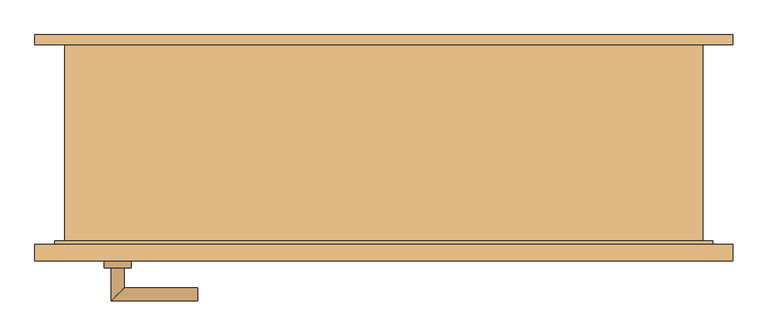
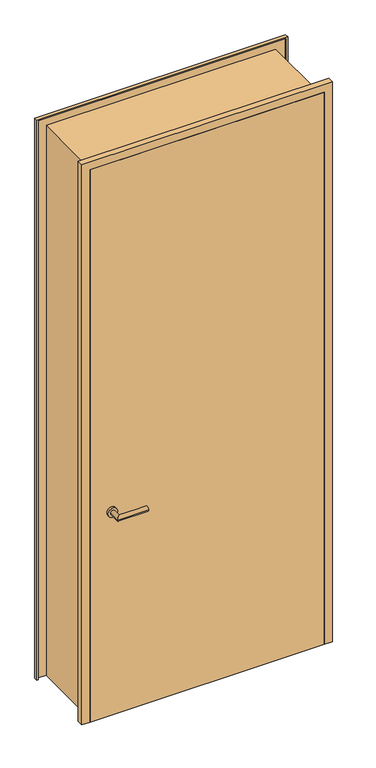
"""IFC4 building model written with IfcOpenShell, lengths in millimetres: door geometry, Drehflügel 1-flg - Stahlzarge : Holztüre 1,0 x 2,45."""

import ifcopenshell
import ifcopenshell.guid

model = None  # the IFC model being written
_history = None  # IfcOwnerHistory: only IFC2X3 demands one
_inside = {}  # id of a spatial element -> (the spatial element, [elements in it])
_under = {}  # id of a project, library or spatial element -> (it, [spatial elements below it])
_declared = {}  # id of a project -> (the project, [libraries it declares])
_typed = {}  # id of a type object -> (the type object, [elements of that type])
_made_of = {}  # id of a material, layer set ... -> (it, [elements and type objects made of it])


def new_model(schema):
    """Start an empty IFC model of exactly this schema.

    Asked for "IFC4X3", IfcOpenShell would pick the latest addendum, in which some entities
    have other attributes; the version numbers below select the first issue.
    IFC2X3 requires an IfcOwnerHistory on every rooted entity: one is made here for all.
    """
    global model, _history
    if schema == "IFC4X3":
        model = ifcopenshell.file(schema_version=(4, 3, 0, 0))
    else:
        model = ifcopenshell.file(schema=schema)
    _inside.clear()
    _under.clear()
    _declared.clear()
    _typed.clear()
    _made_of.clear()
    _history = None
    if model.schema == "IFC2X3":
        org = make("IfcOrganization", Name="unknown")
        user = make(
            "IfcPersonAndOrganization",
            ThePerson=make("IfcPerson", FamilyName="unknown"),
            TheOrganization=org,
        )
        app = make(
            "IfcApplication",
            ApplicationDeveloper=org,
            Version="unknown",
            ApplicationFullName="unknown",
            ApplicationIdentifier="unknown",
        )
        _history = make(
            "IfcOwnerHistory",
            OwningUser=user,
            OwningApplication=app,
            ChangeAction="ADDED",
            CreationDate=0,
        )
    return model


def make(cls, **values):
    """One entity of the class cls with the attributes given. An attribute that is None is left unset."""
    return model.create_entity(
        cls, **{name: value for name, value in values.items() if value is not None}
    )


def rooted(cls, **values):
    """An entity with a GlobalId (a new one), such as an element, a storey or a relation."""
    return make(cls, GlobalId=ifcopenshell.guid.new(), OwnerHistory=_history, **values)


def si_unit(unit_type, name, prefix=None):
    """IfcSIUnit, for example si_unit("LENGTHUNIT", "METRE", prefix="MILLI")."""
    return make("IfcSIUnit", UnitType=unit_type, Prefix=prefix, Name=name)


def assignment(units):
    """IfcUnitAssignment: the units of a project."""
    return None if units is None else make("IfcUnitAssignment", Units=units)


def point(xyz):
    """IfcCartesianPoint."""
    return None if xyz is None else make("IfcCartesianPoint", Coordinates=xyz)


def direction(xyz):
    """IfcDirection."""
    return None if xyz is None else make("IfcDirection", DirectionRatios=xyz)


def frame(location, z_axis=None, x_axis=None):
    """IfcAxis2Placement3D, a coordinate frame: its origin and axes. An axis left out is left unset."""
    return make(
        "IfcAxis2Placement3D",
        Location=point(location),
        Axis=direction(z_axis),
        RefDirection=direction(x_axis),
    )


def frame_2d(location, x_axis=None):
    """IfcAxis2Placement2D, a coordinate frame in the plane: its origin and x axis."""
    return make(
        "IfcAxis2Placement2D", Location=point(location), RefDirection=direction(x_axis)
    )


def origin():
    """The frame at (0, 0, 0) with its axes left unset."""
    return frame((0.0, 0.0, 0.0))


def place(relative_to, where):
    """IfcLocalPlacement: puts the frame where relative to a parent placement (None: the world)."""
    return make(
        "IfcLocalPlacement", PlacementRelTo=relative_to, RelativePlacement=where
    )


def context(
    kind, dimensions, precision=None, world=None, true_north=None, identifier=None
):
    """IfcGeometricRepresentationContext, for example the 3D "Model" context."""
    return make(
        "IfcGeometricRepresentationContext",
        ContextIdentifier=identifier,
        ContextType=kind,
        CoordinateSpaceDimension=dimensions,
        Precision=precision,
        WorldCoordinateSystem=world,
        TrueNorth=true_north,
    )


def project(units=None, contexts=None):
    """IfcProject with its units and contexts."""
    return rooted(
        "IfcProject",
        Name="project",
        RepresentationContexts=contexts,
        UnitsInContext=assignment(units),
    )


def spatial(cls, under=None, at=None, **own):
    """A site, building, storey or space (cls), placed at a placement, below another one or the project."""
    s = rooted(cls, ObjectPlacement=at, **own)
    if under is not None:
        _under.setdefault(under.id(), (under, []))[1].append(s)
    return s


def polyline(points):
    """IfcPolyline through the points."""
    return make("IfcPolyline", Points=[point(p) for p in points])


def circle_curve(where, radius):
    """IfcCircle in the frame where."""
    return make("IfcCircle", Position=where, Radius=radius)


def ellipse_curve(where, semi_axis1, semi_axis2):
    """IfcEllipse in the frame where."""
    return make(
        "IfcEllipse", Position=where, SemiAxis1=semi_axis1, SemiAxis2=semi_axis2
    )


def trimmed(basis, trim1, trim2, sense, master):
    """IfcTrimmedCurve: the piece of a basis curve between two trims."""
    return make(
        "IfcTrimmedCurve",
        BasisCurve=basis,
        Trim1=trim1,
        Trim2=trim2,
        SenseAgreement=sense,
        MasterRepresentation=master,
    )


def segment(curve, same_sense, transition):
    """IfcCompositeCurveSegment."""
    return make(
        "IfcCompositeCurveSegment",
        Transition=transition,
        SameSense=same_sense,
        ParentCurve=curve,
    )


def composite_curve(segments, self_intersect=None):
    """IfcCompositeCurve: segments joined end to end."""
    return make("IfcCompositeCurve", Segments=segments, SelfIntersect=self_intersect)


def outline(outer, holes=None, kind="AREA"):
    """IfcArbitraryClosedProfileDef: a profile drawn as a closed curve; with holes, ...WithVoids."""
    if holes is None:
        return make("IfcArbitraryClosedProfileDef", ProfileType=kind, OuterCurve=outer)
    return make(
        "IfcArbitraryProfileDefWithVoids",
        ProfileType=kind,
        OuterCurve=outer,
        InnerCurves=holes,
    )


def extrude(swept, where, along, depth):
    """IfcExtrudedAreaSolid: the profile swept, set in the frame where, extruded along a direction by depth."""
    return make(
        "IfcExtrudedAreaSolid",
        SweptArea=swept,
        Position=where,
        ExtrudedDirection=direction(along),
        Depth=depth,
    )


def faces_of(points, faces, orient=None, outer=None):
    """IfcFace entities. A face is a list of loops; a loop is a list of indices into points, from 0.

    orient and outer hold one flag for each loop. By default every Orientation is true, the
    first loop of a face is its IfcFaceOuterBound and the others are IfcFaceBound.
    """
    made = []
    for i, loops in enumerate(faces):
        bounds = []
        for j, loop in enumerate(loops):
            is_outer = j == 0 if outer is None else outer[i][j]
            bounds.append(
                make(
                    "IfcFaceOuterBound" if is_outer else "IfcFaceBound",
                    Bound=make("IfcPolyLoop", Polygon=[points[k] for k in loop]),
                    Orientation=True if orient is None else orient[i][j],
                )
            )
        made.append(make("IfcFace", Bounds=bounds))
    return made


def faceted_brep(points, faces, orient=None, outer=None, voids=None):
    """IfcFacetedBrep: a solid bounded by flat faces; with voids (closed shells), ...WithVoids."""
    shared = [point(p) for p in points]
    hull = make("IfcClosedShell", CfsFaces=faces_of(shared, faces, orient, outer))
    if voids is None:
        return make("IfcFacetedBrep", Outer=hull)
    return make(
        "IfcFacetedBrepWithVoids",
        Outer=hull,
        Voids=[
            make(cls, CfsFaces=faces_of(shared, fs, o, b)) for cls, fs, o, b in voids
        ],
    )


def shape(context_of_items, identifier, shape_type, items):
    """IfcShapeRepresentation: the items that make up one representation, for example the "Body"."""
    return make(
        "IfcShapeRepresentation",
        ContextOfItems=context_of_items,
        RepresentationIdentifier=identifier,
        RepresentationType=shape_type,
        Items=items,
    )


def source(mapping_origin, context_of_items, identifier, shape_type, items):
    """IfcRepresentationMap: a shape defined once, which mapped items show again and again."""
    return make(
        "IfcRepresentationMap",
        MappingOrigin=mapping_origin,
        MappedRepresentation=shape(context_of_items, identifier, shape_type, items),
    )


def transform(
    local_origin,
    x_axis=None,
    y_axis=None,
    z_axis=None,
    scale=None,
    scale2=None,
    scale3=None,
    uniform=True,
):
    """IfcCartesianTransformationOperator3D, or its non-uniform kind. x_axis, y_axis, z_axis: its Axis1, 2, 3."""
    if uniform:
        return make(
            "IfcCartesianTransformationOperator3D",
            Axis1=direction(x_axis),
            Axis2=direction(y_axis),
            LocalOrigin=point(local_origin),
            Scale=scale,
            Axis3=direction(z_axis),
        )
    return make(
        "IfcCartesianTransformationOperator3DnonUniform",
        Axis1=direction(x_axis),
        Axis2=direction(y_axis),
        LocalOrigin=point(local_origin),
        Scale=scale,
        Axis3=direction(z_axis),
        Scale2=scale2,
        Scale3=scale3,
    )


def mapped(mapping_source, mapping_target):
    """IfcMappedItem: shows the shape of a source again, moved by a transform."""
    return make(
        "IfcMappedItem", MappingSource=mapping_source, MappingTarget=mapping_target
    )


def made_of(thing, what):
    """Note that an element or type object is made of a material, layer set ...; save() writes the relation."""
    if what is not None:
        _made_of.setdefault(what.id(), (what, []))[1].append(thing)
    return thing


def element(
    cls,
    number,
    at=None,
    inside=None,
    cuts=None,
    type_object=None,
    material=None,
    context=None,
    identifier="Body",
    shape_type=None,
    held_by="IfcProductDefinitionShape",
    body=None,
    shapes=None,
    **own,
):
    """One element of the class cls, such as IfcWall. Its Tag is "e" and its number.

    at: its placement. inside: the storey or other place that contains it. cuts: it is an
    opening in that element (IfcRelVoidsElement). A single representation is given by context,
    identifier, shape_type and body (its items); several are given by shapes. held_by: the class
    of the entity that holds the representations. save() writes the other relations.
    """
    e = rooted(cls, Tag="e%d" % number, ObjectPlacement=at, **own)
    if body is not None:
        shapes = [shape(context, identifier, shape_type, body)]
    if shapes is not None:
        e.Representation = make(held_by, Representations=shapes)
    if inside is not None:
        _inside.setdefault(inside.id(), (inside, []))[1].append(e)
    if cuts is not None:
        rooted(
            "IfcRelVoidsElement", RelatingBuildingElement=cuts, RelatedOpeningElement=e
        )
    if type_object is not None:
        _typed.setdefault(type_object.id(), (type_object, []))[1].append(e)
    return made_of(e, material)


def aggregate(whole, parts):
    """IfcRelAggregates: a whole, such as a stair, and the parts it consists of."""
    return rooted("IfcRelAggregates", RelatingObject=whole, RelatedObjects=parts)


def save(model, path):
    """Write the relations noted so far, then the file.

    IfcRelAggregates (storeys below a building ...), IfcRelContainedInSpatialStructure (elements
    in a storey), IfcRelDefinesByType, IfcRelAssociatesMaterial and IfcRelDeclares: one each for
    every whole, place, type object, material and project.
    """
    for whole, parts in _under.values():
        aggregate(whole, parts)
    for where, things in _inside.values():
        rooted(
            "IfcRelContainedInSpatialStructure",
            RelatedElements=things,
            RelatingStructure=where,
        )
    for kind, things in _typed.values():
        rooted("IfcRelDefinesByType", RelatedObjects=things, RelatingType=kind)
    for what, things in _made_of.values():
        rooted("IfcRelAssociatesMaterial", RelatedObjects=things, RelatingMaterial=what)
    for by, libraries in _declared.values():
        rooted("IfcRelDeclares", RelatingContext=by, RelatedDefinitions=libraries)
    model.write(path)


def plane_surface(at):
    """IfcPlane: the flat surface through the origin of the frame at, square to its z axis."""
    return make("IfcPlane", Position=at)


def cylinder_surface(at, radius):
    """IfcCylindricalSurface: all points at the distance radius from the z axis of the frame at."""
    return make("IfcCylindricalSurface", Position=at, Radius=radius)


def advanced_brep(points, edges, surfaces, faces):
    """IfcAdvancedBrep: a solid bounded by faces that lie on surfaces and meet in shared edges.

    An edge is (start, end): straight between two places in points (the first is 0);
    or (start, end, curve); or (start, end, curve, False) where it runs against its curve.
    A face is (place in surfaces, loops), or (place, loops, False) where it looks against
    its surface's normal. A loop lists edges by number (the first is 1), with a minus sign
    where the edge is run from its end to its start. The first loop is the outer one.
    """
    corners = [point(p) for p in points]
    vertices = [make("IfcVertexPoint", VertexGeometry=c) for c in corners]
    made = []
    for start, end, *more in edges:
        made.append(
            make(
                "IfcEdgeCurve",
                EdgeStart=vertices[start],
                EdgeEnd=vertices[end],
                EdgeGeometry=more[0] if more else make("IfcPolyline", Points=[corners[start], corners[end]]),
                SameSense=more[1] if len(more) > 1 else True,
            )
        )
    hull = []
    for where, loops, *sense in faces:
        bounds = []
        for j, loop in enumerate(loops):
            ring = [make("IfcOrientedEdge", EdgeElement=made[abs(k) - 1], Orientation=k > 0) for k in loop]
            bounds.append(
                make(
                    "IfcFaceOuterBound" if j == 0 else "IfcFaceBound",
                    Bound=make("IfcEdgeLoop", EdgeList=ring),
                    Orientation=True,
                )
            )
        hull.append(make("IfcAdvancedFace", Bounds=bounds, FaceSurface=surfaces[where], SameSense=sense[0] if sense else True))
    return make("IfcAdvancedBrep", Outer=make("IfcClosedShell", CfsFaces=hull))


def door_fb35d1c2(model_context):
    return source(origin(), model_context, "Body", "SolidModel", [
        advanced_brep(
        [(-410.0, -139.4346141, 1000.0), (-390.0, -139.4346141, 1000.0), (-390.0, -89.4346141, 1000.0), (-410.0, -69.4346141, 1000.0), (-280.0, -69.4346141, 1000.0), (-280.0, -89.4346141, 1000.0)],
        [
            (0, 1, circle_curve(frame((-400.0, -139.4346141, 1000.0), z_axis=(0.0, -1.0, 0.0), x_axis=(1.0, 0.0, 0.0)), 10.0)),
            (1, 0, circle_curve(frame((-400.0, -139.4346141, 1000.0), z_axis=(0.0, -1.0, 0.0), x_axis=(1.0, 0.0, 0.0)), 10.0)),
            (1, 2),
            (2, 3, ellipse_curve(frame((-400.0, -79.4346141, 1000.0), z_axis=(-0.7071067811865385, -0.7071067811865565, 0.0), x_axis=(0.7071067811865563, -0.7071067811865386, 0.0)), 14.1421356, 10.0)),
            (3, 0),
            (3, 2, ellipse_curve(frame((-400.0, -79.4346141, 1000.0), z_axis=(-0.7071067811865385, -0.7071067811865565, 0.0), x_axis=(0.7071067811865563, -0.7071067811865386, 0.0)), 14.1421356, 10.0)),
            (4, 5, circle_curve(frame((-280.0, -79.4346141, 1000.0), z_axis=(1.0, 0.0, 0.0), x_axis=(0.0, -1.0, 0.0)), 10.0)),
            (5, 4, circle_curve(frame((-280.0, -79.4346141, 1000.0), z_axis=(1.0, 0.0, 0.0), x_axis=(0.0, -1.0, 0.0)), 10.0)),
            (2, 5),
            (4, 3),
        ],
        [
            plane_surface(frame((-400.0, -139.4346141, -287.7526403), z_axis=(0.0, -1.0, 0.0), x_axis=(0.0, 0.0, 1.0))),
            cylinder_surface(frame((-400.0, -139.4346141, 1000.0), z_axis=(0.0, -1.0, 0.0), x_axis=(1.0, 0.0, 0.0)), 10.0),
            plane_surface(frame((-280.0, -79.4346141, -287.7526403), z_axis=(1.0, 0.0, 0.0), x_axis=(0.0, 0.0, 1.0))),
            cylinder_surface(frame((-400.0, -79.4346141, 1000.0), z_axis=(-1.0, 0.0, 0.0), x_axis=(0.0, -1.0, 0.0)), 10.0),
        ],
        [
            (0, [[1, 2]]),
            (1, [[3, 4, 5, -2]]),
            (1, [[-5, 6, -3, -1]]),
            (2, [[7, 8]]),
            (3, [[9, -7, 10, -4]]),
            (3, [[-10, -8, -9, -6]]),
        ],
    ),
        advanced_brep(
        [(-390.0, -199.4346141, 1000.0), (-410.0, -199.4346141, 1000.0), (-410.0, -249.4346141, 1000.0), (-390.0, -229.4346141, 1000.0), (-280.0, -229.4346141, 1000.0), (-280.0, -249.4346141, 1000.0)],
        [
            (0, 1, circle_curve(frame((-400.0, -199.4346141, 1000.0), z_axis=(0.0, 1.0, 0.0), x_axis=(-1.0, 0.0, 0.0)), 10.0)),
            (1, 0, circle_curve(frame((-400.0, -199.4346141, 1000.0), z_axis=(0.0, 1.0, 0.0), x_axis=(-1.0, 0.0, 0.0)), 10.0)),
            (1, 2),
            (2, 3, ellipse_curve(frame((-400.0, -239.4346141, 1000.0), z_axis=(-0.7071067811865475, 0.7071067811865475, 0.0), x_axis=(0.7071067811865474, 0.7071067811865476, 0.0)), 14.1421356, 10.0)),
            (3, 0),
            (3, 2, ellipse_curve(frame((-400.0, -239.4346141, 1000.0), z_axis=(-0.7071067811865475, 0.7071067811865475, 0.0), x_axis=(0.7071067811865474, 0.7071067811865476, 0.0)), 14.1421356, 10.0)),
            (4, 5, circle_curve(frame((-280.0, -239.4346141, 1000.0), z_axis=(1.0, 0.0, 0.0), x_axis=(0.0, -1.0, 0.0)), 10.0)),
            (5, 4, circle_curve(frame((-280.0, -239.4346141, 1000.0), z_axis=(1.0, 0.0, 0.0), x_axis=(0.0, -1.0, 0.0)), 10.0)),
            (2, 5),
            (4, 3),
        ],
        [
            plane_surface(frame((-400.0, -199.4346141, -287.7526403), z_axis=(0.0, 1.0, 0.0), x_axis=(0.0, 0.0, 1.0))),
            cylinder_surface(frame((-400.0, -199.4346141, 1000.0), z_axis=(0.0, 1.0, 0.0), x_axis=(-1.0, 0.0, 0.0)), 10.0),
            plane_surface(frame((-280.0, -239.4346141, -287.7526403), z_axis=(1.0, 0.0, 0.0), x_axis=(0.0, 0.0, 1.0))),
            cylinder_surface(frame((-400.0, -239.4346141, 1000.0), z_axis=(-1.0, 0.0, 0.0), x_axis=(0.0, -1.0, 0.0)), 10.0),
        ],
        [
            (0, [[1, 2]]),
            (1, [[3, 4, 5, -2]]),
            (1, [[-5, 6, -3, -1]]),
            (2, [[7, 8]]),
            (3, [[9, -7, 10, -4]]),
            (3, [[-10, -8, -9, -6]]),
        ],
    ),
        extrude(outline(composite_curve([segment(trimmed(circle_curve(frame_2d((1000.0, -400.0)), 20.0), [point((1000.0, -420.0))], [point((1000.0, -380.0))], False, "CARTESIAN"), True, "CONTINUOUS"), segment(trimmed(circle_curve(frame_2d((1000.0, -400.0)), 20.0), [point((1000.0, -380.0))], [point((1000.0, -420.0))], False, "CARTESIAN"), True, "CONTINUOUS")], self_intersect=False)), frame((0.0, -139.4346141, 0.0), z_axis=(0.0, 1.0, 0.0), x_axis=(0.0, 0.0, 1.0)), (0.0, 0.0, 1.0), 10.0),
        extrude(outline(composite_curve([segment(trimmed(circle_curve(frame_2d((1000.0, -400.0)), 20.0), [point((1000.0, -420.0))], [point((1000.0, -380.0))], False, "CARTESIAN"), True, "CONTINUOUS"), segment(trimmed(circle_curve(frame_2d((1000.0, -400.0)), 20.0), [point((1000.0, -380.0))], [point((1000.0, -420.0))], False, "CARTESIAN"), True, "CONTINUOUS")], self_intersect=False)), frame((0.0, -199.4346141, 0.0), z_axis=(0.0, 1.0, 0.0), x_axis=(0.0, 0.0, 1.0)), (0.0, 0.0, 1.0), 10.0),
        extrude(outline(polyline([(490.0, -164.4346141), (490.0, -189.4346141), (-490.0, -189.4346141), (-490.0, -164.4346141), (490.0, -164.4346141)])), frame((0.0, 0.0, 100.0), z_axis=(0.0, 0.0, 1.0), x_axis=(1.0, 0.0, 0.0)), (0.0, 0.0, 1.0), 2440.0),
        faceted_brep([(524.4603207, 150.5653859, 100.0), (524.4603207, 135.5653859, 100.0), (519.4603207, 135.5653859, 100.0), (519.4603207, 145.5653859, 100.0), (480.0, 145.5653859, 100.0), (480.0, -159.4346141, 100.0), (495.0, -159.4346141, 100.0), (495.0, -184.4346141, 100.0), (519.4603207, -184.4346141, 100.0), (519.4603207, -164.4346141, 100.0), (524.4603207, -164.4346141, 100.0), (524.4603207, -189.4346141, 100.0), (490.0, -189.4346141, 100.0), (490.0, -164.4346141, 100.0), (475.0, -164.4346141, 100.0), (475.0, 150.5653859, 100.0), (475.0, 150.5653859, 2525.0), (-475.0, 150.5653859, 2525.0), (-475.0, 150.5653859, 100.0), (-524.4603207, 150.5653859, 100.0), (-524.4603207, 150.5653859, 2574.4603207), (524.4603207, 150.5653859, 2574.4603207), (475.0, -164.4346141, 2525.0), (490.0, -164.4346141, 2540.0), (-490.0, -164.4346141, 2540.0), (-490.0, -164.4346141, 100.0), (-475.0, -164.4346141, 100.0), (-475.0, -164.4346141, 2525.0), (490.0, -189.4346141, 2540.0), (524.4603207, -189.4346141, 2574.4603207), (-524.4603207, -189.4346141, 2574.4603207), (-524.4603207, -189.4346141, 100.0), (-490.0, -189.4346141, 100.0), (-490.0, -189.4346141, 2540.0), (524.4603207, -164.4346141, 2574.4603207), (519.4603207, -164.4346141, 2569.4603207), (-519.4603207, -164.4346141, 2569.4603207), (-519.4603207, -164.4346141, 100.0), (-524.4603207, -164.4346141, 100.0), (-524.4603207, -164.4346141, 2574.4603207), (519.4603207, -184.4346141, 2569.4603207), (495.0, -184.4346141, 2545.0), (-495.0, -184.4346141, 2545.0), (-495.0, -184.4346141, 100.0), (-519.4603207, -184.4346141, 100.0), (-519.4603207, -184.4346141, 2569.4603207), (495.0, -159.4346141, 2545.0), (480.0, -159.4346141, 2530.0), (-480.0, -159.4346141, 2530.0), (-480.0, -159.4346141, 100.0), (-495.0, -159.4346141, 100.0), (-495.0, -159.4346141, 2545.0), (480.0, 145.5653859, 2530.0), (519.4603207, 145.5653859, 2569.4603207), (-519.4603207, 145.5653859, 2569.4603207), (-519.4603207, 145.5653859, 100.0), (-480.0, 145.5653859, 100.0), (-480.0, 145.5653859, 2530.0), (519.4603207, 135.5653859, 2569.4603207), (524.4603207, 135.5653859, 2574.4603207), (-524.4603207, 135.5653859, 2574.4603207), (-524.4603207, 135.5653859, 100.0), (-519.4603207, 135.5653859, 100.0), (-519.4603207, 135.5653859, 2569.4603207)], [[[0, 1, 2, 3, 4, 5, 6, 7, 8, 9, 10, 11, 12, 13, 14, 15]], [[15, 16, 17, 18, 19, 20, 21, 0]], [[14, 22, 16, 15]], [[13, 23, 24, 25, 26, 27, 22, 14]], [[12, 28, 23, 13]], [[11, 29, 30, 31, 32, 33, 28, 12]], [[10, 34, 29, 11]], [[9, 35, 36, 37, 38, 39, 34, 10]], [[8, 40, 35, 9]], [[7, 41, 42, 43, 44, 45, 40, 8]], [[6, 46, 41, 7]], [[5, 47, 48, 49, 50, 51, 46, 6]], [[4, 52, 47, 5]], [[3, 53, 54, 55, 56, 57, 52, 4]], [[2, 58, 53, 3]], [[1, 59, 60, 61, 62, 63, 58, 2]], [[0, 21, 59, 1]], [[20, 19, 61, 60]], [[19, 18, 26, 25, 32, 31, 38, 37, 44, 43, 50, 49, 56, 55, 62, 61]], [[27, 26, 18, 17]], [[33, 32, 25, 24]], [[39, 38, 31, 30]], [[45, 44, 37, 36]], [[51, 50, 43, 42]], [[57, 56, 49, 48]], [[63, 62, 55, 54]], [[22, 27, 17, 16]], [[28, 33, 24, 23]], [[34, 39, 30, 29]], [[40, 45, 36, 35]], [[46, 51, 42, 41]], [[52, 57, 48, 47]], [[58, 63, 54, 53]], [[21, 20, 60, 59]]]),
    ])


if __name__ == "__main__":
    model = new_model("IFC4")
    model_context = context("Model", 3, world=origin())
    ifc_project = project(units=[si_unit("LENGTHUNIT", "METRE", prefix="MILLI")], contexts=[model_context])
    site = spatial("IfcSite", under=ifc_project)
    building = spatial("IfcBuilding", under=site)
    placement = place(None, origin())
    door_shape = door_fb35d1c2(model_context)
    element("IfcDoor", 1, ObjectType="Drehflügel 1-flg - Stahlzarge : Holztüre 1,0 x 2,45", at=placement, inside=building, context=model_context, shape_type="MappedRepresentation", body=[
        mapped(door_shape, transform((0.0, 0.0, 0.0), x_axis=(1.0, 0.0, 0.0), y_axis=(0.0, 1.0, 0.0), z_axis=(0.0, 0.0, 1.0))),
    ])
    save(model, "model.ifc")

# Revit data of these elements
# Type "Drehflügel 1-flg - Stahlzarge : Holztüre 1,0 x 2,45"
#   Type Mark = "23"
#   Operation = "SingleSwingRight"
#   Keynote = "16.03"
#   Analytic Construction = "Metall"
#   Thermal Resistance (R) = 0.270117 (m²·K)/W
#   Heat Transfer Coefficient (U) = 3.7021 W/(m²·K)
#   Rough Width = 1.000 m
#   Rough Height [instance default] = 2.550 m
#   Höhe Türgriff [instance default] = 0.900 m
#   Height = 2.450 m
#   Fußbodenaufbau [instance default] = 0.100 m
#   Width = 1.000 m
#   Sichtbarkeit Sturzlinien [instance default] = yes
#   Türgriff auswählen [instance default] = element 221079
#   Türgriff [instance default] = none
#   Türflügel [instance default] = none
#   Rahmen/Pfosten [instance default] = Metall - Lackiert - Grau
#   Visual Light Transmittance = 0
#   Solar Heat Gain Coefficient = 0
#   Function = (empty or 0)
#   Wall Closure = (empty or 0)
# Element 1 (IfcDoor, "Drehflügel 1-flg - Stahlzarge : Holztüre 1,0 x 2,45")
#   Rahmen/Pfosten = Holz - Eiche
#   Materials on its faces: "Holz - Eiche", "Metall - Chrom", "Holz - Birke"
# Materials
#   "Metall - Lackiert - Grau": class "Farbe 1", colour RGB 98 98 98, transparency 0, Cost = 0
#   "Holz - Eiche": class "Holz", colour RGB 151 89 53, transparency 0, Cost = 0
#   "Metall - Chrom": class "Metall", colour RGB 247 247 247, transparency 0, Cost = 0
#   "Holz - Birke": class "Holz", colour RGB 213 164 103, transparency 0, Cost = 0
